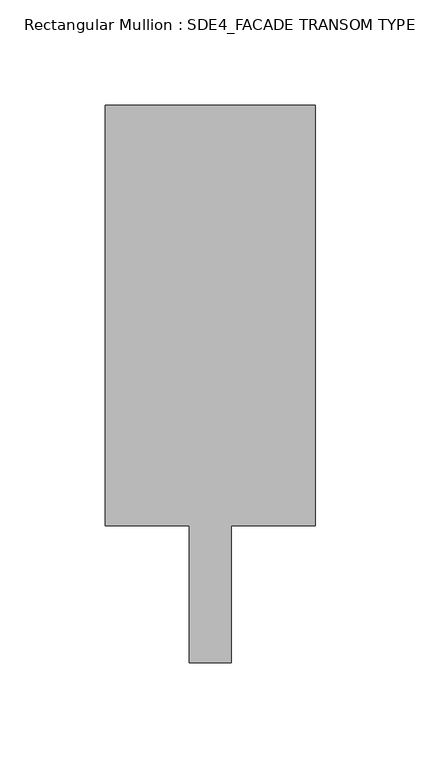
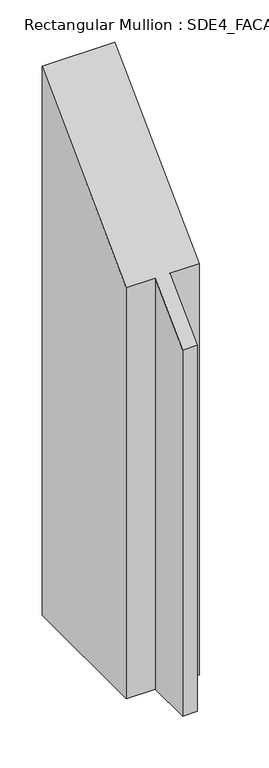
"""IFC4 building model written with IfcOpenShell, lengths in millimetres: member geometry, Rectangular Mullion : SDE4_FACADE TRANSOM TYPE 2."""

from ifc_helpers import new_model, si_unit, origin, place, context, project, spatial, faceted_brep, source, transform, mapped, element, save


def rectangular_mullion_sde4_facade_transom_type_2_576b8cad(model_context):
    return source(origin(), model_context, "Body", "Brep", [
        faceted_brep([(50.0, 132.5, -663.5506048), (50.0, -67.5, -663.5506048), (10.0, -67.5, -663.5506048), (10.0, -132.5, -663.5506048), (-10.0, -132.5, -663.5506048), (-10.0, -67.5, -663.5506048), (-50.0, -67.5, -663.5506048), (-50.0, 132.5, -663.5506048), (-50.0, 132.5, 132.5), (50.0, 132.5, 132.5), (-50.0, -67.5, -67.5), (-10.0, -67.5, -67.5), (-10.0, -132.5, -132.5), (10.0, -132.5, -132.5), (10.0, -67.5, -67.5), (50.0, -67.5, -67.5)], [[[0, 1, 2, 3, 4, 5, 6, 7]], [[8, 9, 0, 7]], [[10, 8, 7, 6]], [[11, 10, 6, 5]], [[12, 11, 5, 4]], [[13, 12, 4, 3]], [[14, 13, 3, 2]], [[15, 14, 2, 1]], [[9, 15, 1, 0]], [[9, 8, 10, 11, 12, 13, 14, 15]]]),
    ])


if __name__ == "__main__":
    model = new_model("IFC4")
    model_context = context("Model", 3, world=origin())
    ifc_project = project(units=[si_unit("LENGTHUNIT", "METRE", prefix="MILLI")], contexts=[model_context])
    site = spatial("IfcSite", under=ifc_project)
    building = spatial("IfcBuilding", under=site)
    placement = place(None, origin())
    rectangular_mullion_sde4_facade_transom_type_2_shape = rectangular_mullion_sde4_facade_transom_type_2_576b8cad(model_context)
    element("IfcMember", 1, ObjectType="Rectangular Mullion : SDE4_FACADE TRANSOM TYPE 2", at=placement, inside=building, context=model_context, shape_type="MappedRepresentation", body=[
        mapped(rectangular_mullion_sde4_facade_transom_type_2_shape, transform((0.0, 0.0, 0.0), x_axis=(1.0, 0.0, 0.0), y_axis=(0.0, 1.0, 0.0), z_axis=(0.0, 0.0, 1.0))),
    ])
    save(model, "model.ifc")

# Revit data of these elements
# Type "Rectangular Mullion : SDE4_FACADE TRANSOM TYPE 2"
#   built-in parameter 1007322 = 0.869423 (stored number, unit not read)
#   built-in parameter 1007321 = 0.164042 (stored number, unit not read)
#   built-in parameter 1007320 = 0.164042 (stored number, unit not read)
